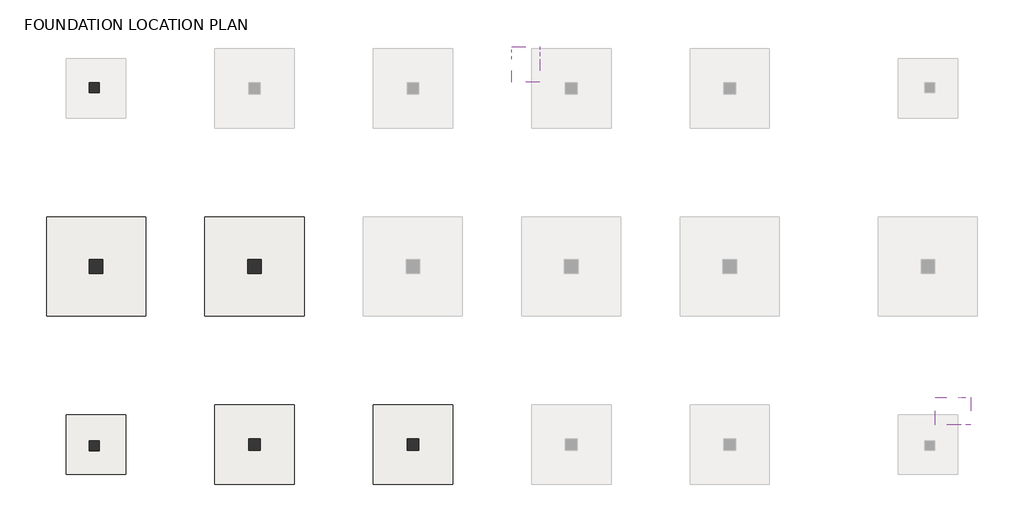
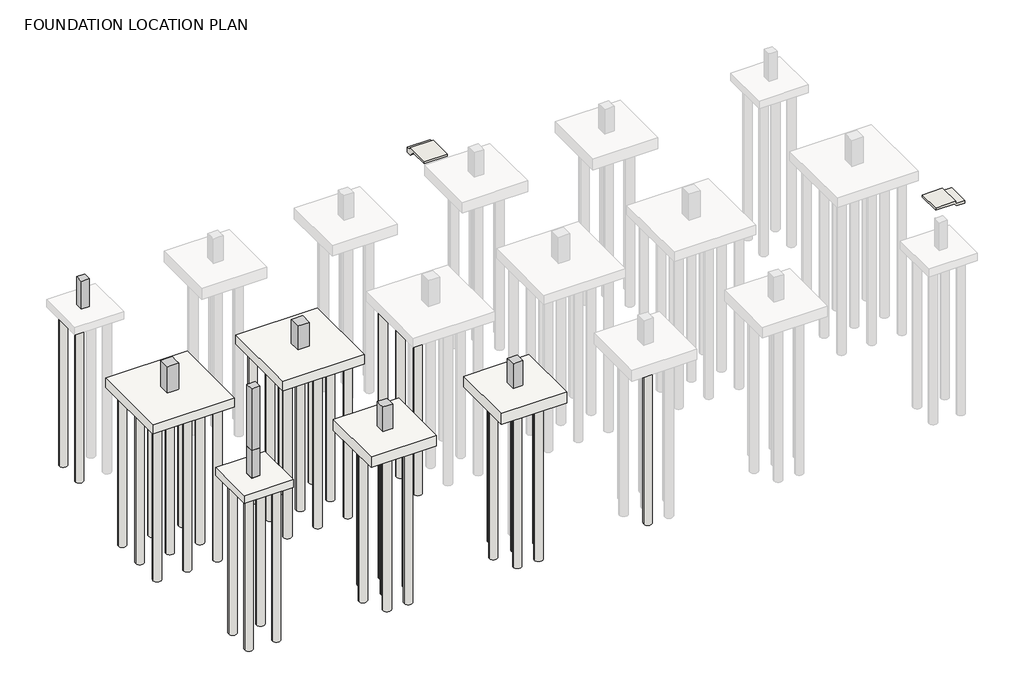
# One storey, part 1 of 3: 46 slabs, 7 columns, 2 walls.
# Revit data of these elements (continued)
# Materials (continued)
#   "A03AC035-00001_Form Work (3 times in use)_Flat": class "Wood", colour RGB 149 120 74, transparency 0, Description = "Plywood", W00) Work Master Code = "A03AC035-00001", W01) Work Master_Lv1 = "Concrete Work", W02) Work Master_Lv2 = "Substructure Work", W03) Work Master_Spec.1 = "Form Work (3 times in use)", W04) Work Master_Spec.2 = "Flat Form", W05) Work Master_Spec.3 = "Dressed Lumber, Plywood or Steel Form(Wood Planks are not Allowed) incl. Chamfer", Cost = 0
#   "A03AC032-00007_Structural Concrete_Type1_25MPa-30Mpa": class "Concrete", colour RGB 176 176 176, transparency 0, Keynote = "09910.A1", Description = "Reinf. Conc.", W00) Work Master Code = "A03AC032-00007", W01) Work Master_Lv1 = "Concrete Work", W02) Work Master_Lv2 = "Substructure Work", W03) Work Master_Spec.1 = "Structural Concrete", W04) Work Master_Spec.2 = "Cement Type-1", W05) Work Master_Spec.3 = "25MPa < F'c (Cylinder Strength) ≤ 30MPa", Cost = 0
#   "A02AA014-00001_Piling Work_Reinforced Concrete Pile(Round Type)_Direct Driving": class "Concrete", colour RGB 176 176 176, transparency 0, Keynote = "09910.A1", Description = "Reinf. Conc.", Cost = 0
#   "A03AD032-00007_Structural Concrete_25MPa-30MPa": class "Concrete", colour RGB 176 176 176, transparency 0, Keynote = "09910.A1", Description = "ACRYLIC EMULSION PAINT ON\nFAIR FACED CONC.", W00) Work Master Code = "A03AD032-00007", W01) Work Master_Lv1 = "Concrete Work", W02) Work Master_Lv2 = "Superstructure Work", W03) Work Master_Spec.1 = "Structural Concrete", W04) Work Master_Spec.2 = "Cement Type-1", W05) Work Master_Spec.3 = "25MPa < F'c (Cylinder Strength) ≤ 30MPa", Cost = 0
